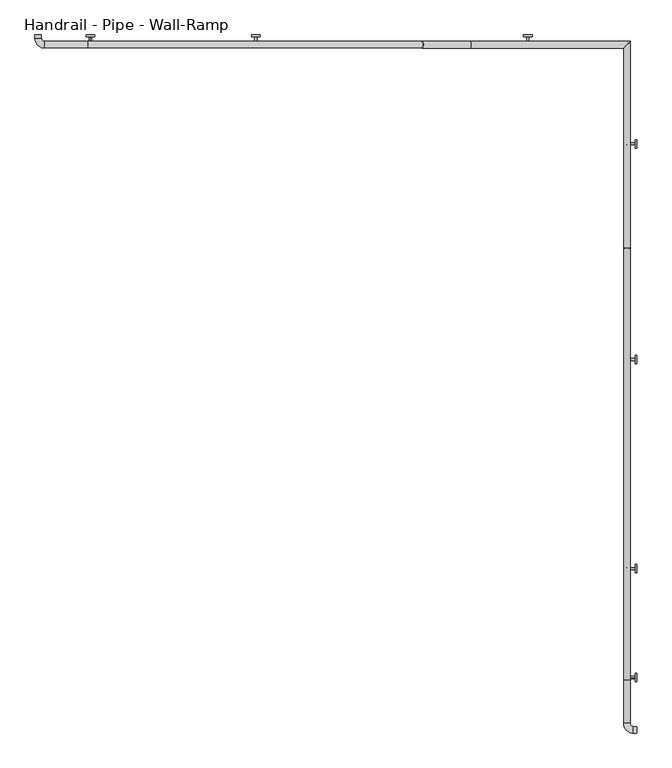
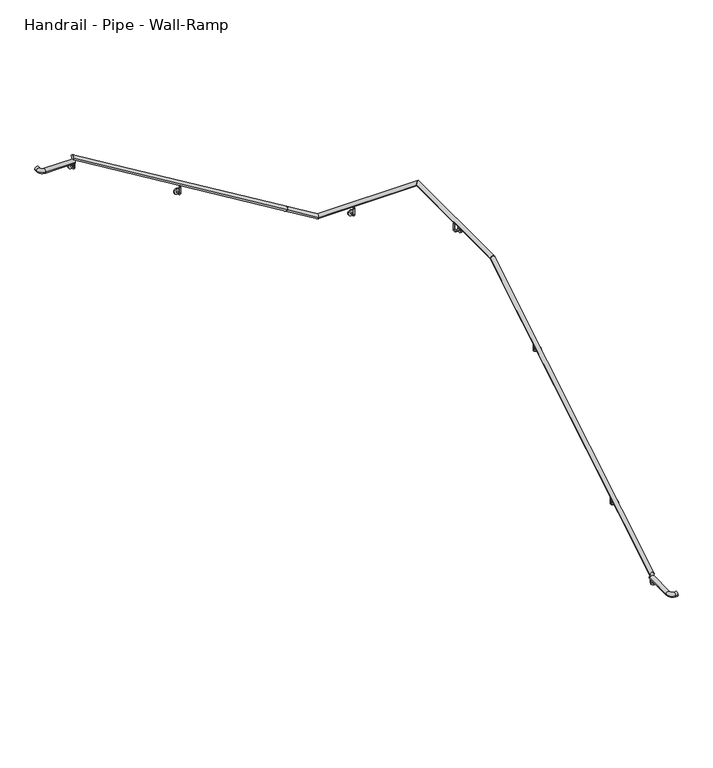
"""IFC4 building model written with IfcOpenShell, lengths in millimetres: railing geometry, Handrail - Pipe - Wall-Ramp."""

import ifcopenshell
import ifcopenshell.guid

model = None  # the IFC model being written
_history = None  # IfcOwnerHistory: only IFC2X3 demands one
_inside = {}  # id of a spatial element -> (the spatial element, [elements in it])
_under = {}  # id of a project, library or spatial element -> (it, [spatial elements below it])
_declared = {}  # id of a project -> (the project, [libraries it declares])
_typed = {}  # id of a type object -> (the type object, [elements of that type])
_made_of = {}  # id of a material, layer set ... -> (it, [elements and type objects made of it])


def new_model(schema):
    """Start an empty IFC model of exactly this schema.

    Asked for "IFC4X3", IfcOpenShell would pick the latest addendum, in which some entities
    have other attributes; the version numbers below select the first issue.
    IFC2X3 requires an IfcOwnerHistory on every rooted entity: one is made here for all.
    """
    global model, _history
    if schema == "IFC4X3":
        model = ifcopenshell.file(schema_version=(4, 3, 0, 0))
    else:
        model = ifcopenshell.file(schema=schema)
    _inside.clear()
    _under.clear()
    _declared.clear()
    _typed.clear()
    _made_of.clear()
    _history = None
    if model.schema == "IFC2X3":
        org = make("IfcOrganization", Name="unknown")
        user = make(
            "IfcPersonAndOrganization",
            ThePerson=make("IfcPerson", FamilyName="unknown"),
            TheOrganization=org,
        )
        app = make(
            "IfcApplication",
            ApplicationDeveloper=org,
            Version="unknown",
            ApplicationFullName="unknown",
            ApplicationIdentifier="unknown",
        )
        _history = make(
            "IfcOwnerHistory",
            OwningUser=user,
            OwningApplication=app,
            ChangeAction="ADDED",
            CreationDate=0,
        )
    return model


def make(cls, **values):
    """One entity of the class cls with the attributes given. An attribute that is None is left unset."""
    return model.create_entity(
        cls, **{name: value for name, value in values.items() if value is not None}
    )


def rooted(cls, **values):
    """An entity with a GlobalId (a new one), such as an element, a storey or a relation."""
    return make(cls, GlobalId=ifcopenshell.guid.new(), OwnerHistory=_history, **values)


def si_unit(unit_type, name, prefix=None):
    """IfcSIUnit, for example si_unit("LENGTHUNIT", "METRE", prefix="MILLI")."""
    return make("IfcSIUnit", UnitType=unit_type, Prefix=prefix, Name=name)


def assignment(units):
    """IfcUnitAssignment: the units of a project."""
    return None if units is None else make("IfcUnitAssignment", Units=units)


def point(xyz):
    """IfcCartesianPoint."""
    return None if xyz is None else make("IfcCartesianPoint", Coordinates=xyz)


def direction(xyz):
    """IfcDirection."""
    return None if xyz is None else make("IfcDirection", DirectionRatios=xyz)


def frame(location, z_axis=None, x_axis=None):
    """IfcAxis2Placement3D, a coordinate frame: its origin and axes. An axis left out is left unset."""
    return make(
        "IfcAxis2Placement3D",
        Location=point(location),
        Axis=direction(z_axis),
        RefDirection=direction(x_axis),
    )


def frame_2d(location, x_axis=None):
    """IfcAxis2Placement2D, a coordinate frame in the plane: its origin and x axis."""
    return make(
        "IfcAxis2Placement2D", Location=point(location), RefDirection=direction(x_axis)
    )


def origin():
    """The frame at (0, 0, 0) with its axes left unset."""
    return frame((0.0, 0.0, 0.0))


def place(relative_to, where):
    """IfcLocalPlacement: puts the frame where relative to a parent placement (None: the world)."""
    return make(
        "IfcLocalPlacement", PlacementRelTo=relative_to, RelativePlacement=where
    )


def context(
    kind, dimensions, precision=None, world=None, true_north=None, identifier=None
):
    """IfcGeometricRepresentationContext, for example the 3D "Model" context."""
    return make(
        "IfcGeometricRepresentationContext",
        ContextIdentifier=identifier,
        ContextType=kind,
        CoordinateSpaceDimension=dimensions,
        Precision=precision,
        WorldCoordinateSystem=world,
        TrueNorth=true_north,
    )


def project(units=None, contexts=None):
    """IfcProject with its units and contexts."""
    return rooted(
        "IfcProject",
        Name="project",
        RepresentationContexts=contexts,
        UnitsInContext=assignment(units),
    )


def spatial(cls, under=None, at=None, **own):
    """A site, building, storey or space (cls), placed at a placement, below another one or the project."""
    s = rooted(cls, ObjectPlacement=at, **own)
    if under is not None:
        _under.setdefault(under.id(), (under, []))[1].append(s)
    return s


def circle_curve(where, radius):
    """IfcCircle in the frame where."""
    return make("IfcCircle", Position=where, Radius=radius)


def ellipse_curve(where, semi_axis1, semi_axis2):
    """IfcEllipse in the frame where."""
    return make(
        "IfcEllipse", Position=where, SemiAxis1=semi_axis1, SemiAxis2=semi_axis2
    )


def trimmed(basis, trim1, trim2, sense, master):
    """IfcTrimmedCurve: the piece of a basis curve between two trims."""
    return make(
        "IfcTrimmedCurve",
        BasisCurve=basis,
        Trim1=trim1,
        Trim2=trim2,
        SenseAgreement=sense,
        MasterRepresentation=master,
    )


def segment(curve, same_sense, transition):
    """IfcCompositeCurveSegment."""
    return make(
        "IfcCompositeCurveSegment",
        Transition=transition,
        SameSense=same_sense,
        ParentCurve=curve,
    )


def composite_curve(segments, self_intersect=None):
    """IfcCompositeCurve: segments joined end to end."""
    return make("IfcCompositeCurve", Segments=segments, SelfIntersect=self_intersect)


def outline(outer, holes=None, kind="AREA"):
    """IfcArbitraryClosedProfileDef: a profile drawn as a closed curve; with holes, ...WithVoids."""
    if holes is None:
        return make("IfcArbitraryClosedProfileDef", ProfileType=kind, OuterCurve=outer)
    return make(
        "IfcArbitraryProfileDefWithVoids",
        ProfileType=kind,
        OuterCurve=outer,
        InnerCurves=holes,
    )


def extrude(swept, where, along, depth):
    """IfcExtrudedAreaSolid: the profile swept, set in the frame where, extruded along a direction by depth."""
    return make(
        "IfcExtrudedAreaSolid",
        SweptArea=swept,
        Position=where,
        ExtrudedDirection=direction(along),
        Depth=depth,
    )


def shape(context_of_items, identifier, shape_type, items):
    """IfcShapeRepresentation: the items that make up one representation, for example the "Body"."""
    return make(
        "IfcShapeRepresentation",
        ContextOfItems=context_of_items,
        RepresentationIdentifier=identifier,
        RepresentationType=shape_type,
        Items=items,
    )


def source(mapping_origin, context_of_items, identifier, shape_type, items):
    """IfcRepresentationMap: a shape defined once, which mapped items show again and again."""
    return make(
        "IfcRepresentationMap",
        MappingOrigin=mapping_origin,
        MappedRepresentation=shape(context_of_items, identifier, shape_type, items),
    )


def transform(
    local_origin,
    x_axis=None,
    y_axis=None,
    z_axis=None,
    scale=None,
    scale2=None,
    scale3=None,
    uniform=True,
):
    """IfcCartesianTransformationOperator3D, or its non-uniform kind. x_axis, y_axis, z_axis: its Axis1, 2, 3."""
    if uniform:
        return make(
            "IfcCartesianTransformationOperator3D",
            Axis1=direction(x_axis),
            Axis2=direction(y_axis),
            LocalOrigin=point(local_origin),
            Scale=scale,
            Axis3=direction(z_axis),
        )
    return make(
        "IfcCartesianTransformationOperator3DnonUniform",
        Axis1=direction(x_axis),
        Axis2=direction(y_axis),
        LocalOrigin=point(local_origin),
        Scale=scale,
        Axis3=direction(z_axis),
        Scale2=scale2,
        Scale3=scale3,
    )


def mapped(mapping_source, mapping_target):
    """IfcMappedItem: shows the shape of a source again, moved by a transform."""
    return make(
        "IfcMappedItem", MappingSource=mapping_source, MappingTarget=mapping_target
    )


def made_of(thing, what):
    """Note that an element or type object is made of a material, layer set ...; save() writes the relation."""
    if what is not None:
        _made_of.setdefault(what.id(), (what, []))[1].append(thing)
    return thing


def element(
    cls,
    number,
    at=None,
    inside=None,
    cuts=None,
    type_object=None,
    material=None,
    context=None,
    identifier="Body",
    shape_type=None,
    held_by="IfcProductDefinitionShape",
    body=None,
    shapes=None,
    **own,
):
    """One element of the class cls, such as IfcWall. Its Tag is "e" and its number.

    at: its placement. inside: the storey or other place that contains it. cuts: it is an
    opening in that element (IfcRelVoidsElement). A single representation is given by context,
    identifier, shape_type and body (its items); several are given by shapes. held_by: the class
    of the entity that holds the representations. save() writes the other relations.
    """
    e = rooted(cls, Tag="e%d" % number, ObjectPlacement=at, **own)
    if body is not None:
        shapes = [shape(context, identifier, shape_type, body)]
    if shapes is not None:
        e.Representation = make(held_by, Representations=shapes)
    if inside is not None:
        _inside.setdefault(inside.id(), (inside, []))[1].append(e)
    if cuts is not None:
        rooted(
            "IfcRelVoidsElement", RelatingBuildingElement=cuts, RelatedOpeningElement=e
        )
    if type_object is not None:
        _typed.setdefault(type_object.id(), (type_object, []))[1].append(e)
    return made_of(e, material)


def aggregate(whole, parts):
    """IfcRelAggregates: a whole, such as a stair, and the parts it consists of."""
    return rooted("IfcRelAggregates", RelatingObject=whole, RelatedObjects=parts)


def save(model, path):
    """Write the relations noted so far, then the file.

    IfcRelAggregates (storeys below a building ...), IfcRelContainedInSpatialStructure (elements
    in a storey), IfcRelDefinesByType, IfcRelAssociatesMaterial and IfcRelDeclares: one each for
    every whole, place, type object, material and project.
    """
    for whole, parts in _under.values():
        aggregate(whole, parts)
    for where, things in _inside.values():
        rooted(
            "IfcRelContainedInSpatialStructure",
            RelatedElements=things,
            RelatingStructure=where,
        )
    for kind, things in _typed.values():
        rooted("IfcRelDefinesByType", RelatedObjects=things, RelatingType=kind)
    for what, things in _made_of.values():
        rooted("IfcRelAssociatesMaterial", RelatedObjects=things, RelatingMaterial=what)
    for by, libraries in _declared.values():
        rooted("IfcRelDeclares", RelatingContext=by, RelatedDefinitions=libraries)
    model.write(path)


def plane_surface(at):
    """IfcPlane: the flat surface through the origin of the frame at, square to its z axis."""
    return make("IfcPlane", Position=at)


def cylinder_surface(at, radius):
    """IfcCylindricalSurface: all points at the distance radius from the z axis of the frame at."""
    return make("IfcCylindricalSurface", Position=at, Radius=radius)


def revolved_surface(curve, axis_point, axis_direction):
    """IfcSurfaceOfRevolution: the curve turned about the line through axis_point along axis_direction."""
    return make(
        "IfcSurfaceOfRevolution",
        SweptCurve=make("IfcArbitraryOpenProfileDef", ProfileType="CURVE", Curve=curve),
        AxisPosition=make("IfcAxis1Placement", Location=point(axis_point), Axis=direction(axis_direction)),
    )


def advanced_brep(points, edges, surfaces, faces):
    """IfcAdvancedBrep: a solid bounded by faces that lie on surfaces and meet in shared edges.

    An edge is (start, end): straight between two places in points (the first is 0);
    or (start, end, curve); or (start, end, curve, False) where it runs against its curve.
    A face is (place in surfaces, loops), or (place, loops, False) where it looks against
    its surface's normal. A loop lists edges by number (the first is 1), with a minus sign
    where the edge is run from its end to its start. The first loop is the outer one.
    """
    corners = [point(p) for p in points]
    vertices = [make("IfcVertexPoint", VertexGeometry=c) for c in corners]
    made = []
    for start, end, *more in edges:
        made.append(
            make(
                "IfcEdgeCurve",
                EdgeStart=vertices[start],
                EdgeEnd=vertices[end],
                EdgeGeometry=more[0] if more else make("IfcPolyline", Points=[corners[start], corners[end]]),
                SameSense=more[1] if len(more) > 1 else True,
            )
        )
    hull = []
    for where, loops, *sense in faces:
        bounds = []
        for j, loop in enumerate(loops):
            ring = [make("IfcOrientedEdge", EdgeElement=made[abs(k) - 1], Orientation=k > 0) for k in loop]
            bounds.append(
                make(
                    "IfcFaceOuterBound" if j == 0 else "IfcFaceBound",
                    Bound=make("IfcEdgeLoop", EdgeList=ring),
                    Orientation=True,
                )
            )
        hull.append(make("IfcAdvancedFace", Bounds=bounds, FaceSurface=surfaces[where], SameSense=sense[0] if sense else True))
    return make("IfcAdvancedBrep", Outer=make("IfcClosedShell", CfsFaces=hull))


def handrail_pipe_wall_ramp_3ec7286e(model_context):
    return source(origin(), model_context, "Body", "SolidModel", [
        advanced_brep(
        [(-6920.3581077, -11181.433999, 1061.4577857), (-6882.2581077, -11181.433999, 1061.4577857), (-6920.3581077, -8661.5118455, 2588.6833333), (-6882.2581077, -8661.5118455, 2588.6833333)],
        [
            (0, 1, ellipse_curve(frame((-6901.3081077, -11181.433999, 1061.4577857), z_axis=(0.0, -1.0, 0.0), x_axis=(0.0, 0.0, -1.0)), 22.2755476, 19.05)),
            (1, 0, ellipse_curve(frame((-6901.3081077, -11181.433999, 1061.4577857), z_axis=(0.0, -1.0, 0.0), x_axis=(0.0, 0.0, -1.0)), 22.2755476, 19.05)),
            (2, 3, ellipse_curve(frame((-6901.3081077, -8661.5118455, 2588.6833333), z_axis=(0.0, 0.963119367356418, 0.26907449567540415), x_axis=(0.0, 0.26907449567540404, -0.9631193673564179)), 19.7794797, 19.05)),
            (3, 2, ellipse_curve(frame((-6901.3081077, -8661.5118455, 2588.6833333), z_axis=(0.0, 0.963119367356418, 0.26907449567540415), x_axis=(0.0, 0.26907449567540404, -0.9631193673564179)), 19.7794797, 19.05)),
            (0, 2),
            (3, 1),
        ],
        [
            plane_surface(frame((-6901.3081077, -11181.433999, 1083.7333333), z_axis=(0.0, -1.0, 0.0), x_axis=(0.0, 0.0, 1.0))),
            plane_surface(frame((-6901.3081077, -8666.833999, 2607.7333333), z_axis=(0.0, 0.963119367356418, 0.26907449567540415), x_axis=(1.0, 0.0, 0.0))),
            cylinder_surface(frame((-6901.3081077, -11171.5603513, 1067.4418146), z_axis=(0.0, -0.8551978315540538, -0.518301716093285), x_axis=(1.0, 0.0, 0.0)), 19.05),
        ],
        [
            (0, [[1, 2]]),
            (1, [[3, 4]]),
            (2, [[-1, 5, -4, 6]]),
            (2, [[-2, -6, -3, -5]]),
        ],
    ),
        advanced_brep(
        [(-6920.3581077, -8661.5118455, 2588.6833333), (-6882.2581077, -8661.5118455, 2588.6833333), (-6920.3581077, -7498.433999, 2588.6833333), (-6882.2581077, -7460.333999, 2588.6833333)],
        [
            (0, 1, ellipse_curve(frame((-6901.3081077, -8661.5118455, 2588.6833333), z_axis=(0.0, -0.963119367356418, -0.26907449567540415), x_axis=(0.0, -0.2690744956754042, 0.963119367356418)), 19.7794797, 19.05)),
            (1, 0, ellipse_curve(frame((-6901.3081077, -8661.5118455, 2588.6833333), z_axis=(0.0, -0.963119367356418, -0.26907449567540415), x_axis=(0.0, -0.2690744956754042, 0.963119367356418)), 19.7794797, 19.05)),
            (2, 3, ellipse_curve(frame((-6901.3081077, -7479.383999, 2588.6833333), z_axis=(-0.7071067811865462, 0.7071067811865488, 0.0), x_axis=(-0.7071067811865488, -0.7071067811865462, 0.0)), 26.9407684, 19.05)),
            (3, 2, ellipse_curve(frame((-6901.3081077, -7479.383999, 2588.6833333), z_axis=(-0.7071067811865462, 0.7071067811865488, 0.0), x_axis=(-0.7071067811865488, -0.7071067811865462, 0.0)), 26.9407684, 19.05)),
            (0, 2),
            (3, 1),
        ],
        [
            plane_surface(frame((-6901.3081077, -8666.833999, 2607.7333333), z_axis=(0.0, -0.963119367356418, -0.26907449567540415), x_axis=(1.0, 0.0, 0.0))),
            plane_surface(frame((-6901.3081077, -7479.383999, 2607.7333333), z_axis=(-0.7071067811865462, 0.7071067811865488, 0.0), x_axis=(0.7071067811865488, 0.7071067811865462, 0.0))),
            cylinder_surface(frame((-6901.3081077, -8666.833999, 2588.6833333), z_axis=(0.0, -1.0, 0.0), x_axis=(1.0, 0.0, 0.0)), 19.05),
        ],
        [
            (0, [[1, 2]]),
            (1, [[3, 4]]),
            (2, [[-1, 5, -4, 6]]),
            (2, [[-2, -6, -3, -5]]),
        ],
    ),
        advanced_brep(
        [(-6920.3581077, -7498.433999, 2588.6833333), (-6882.2581077, -7460.333999, 2588.6833333), (-7814.6802613, -7498.433999, 2588.6833333), (-7814.6802613, -7460.333999, 2588.6833333), (-8098.6317554, -7498.433999, 2760.775148), (-8098.6317554, -7460.333999, 2760.775148)],
        [
            (0, 1, ellipse_curve(frame((-6901.3081077, -7479.383999, 2588.6833333), z_axis=(0.7071067811865462, -0.7071067811865488, 0.0), x_axis=(0.7071067811865488, 0.7071067811865462, 0.0)), 26.9407684, 19.05)),
            (1, 0, ellipse_curve(frame((-6901.3081077, -7479.383999, 2588.6833333), z_axis=(0.7071067811865462, -0.7071067811865488, 0.0), x_axis=(0.7071067811865488, 0.7071067811865462, 0.0)), 26.9407684, 19.05)),
            (0, 2),
            (2, 3, ellipse_curve(frame((-7814.6802613, -7479.383999, 2588.6833333), z_axis=(0.9631193673564179, 0.0, -0.2690744956754043), x_axis=(0.2690744956754048, 0.0, 0.9631193673564179)), 19.7794797, 19.05)),
            (3, 1),
            (3, 2, ellipse_curve(frame((-7814.6802613, -7479.383999, 2588.6833333), z_axis=(0.9631193673564179, 0.0, -0.2690744956754043), x_axis=(0.2690744956754048, 0.0, 0.9631193673564179)), 19.7794797, 19.05)),
            (4, 5, circle_curve(frame((-8098.6317554, -7479.383999, 2760.775148), z_axis=(-0.8551978315540536, 0.0, 0.5183017160932853), x_axis=(0.0, 1.0, 0.0)), 19.05)),
            (5, 4, circle_curve(frame((-8098.6317554, -7479.383999, 2760.775148), z_axis=(-0.8551978315540536, 0.0, 0.5183017160932853), x_axis=(0.0, 1.0, 0.0)), 19.05)),
            (2, 4),
            (5, 3),
        ],
        [
            plane_surface(frame((-6901.3081077, -7479.383999, 2607.7333333), z_axis=(0.7071067811865462, -0.7071067811865488, 0.0), x_axis=(0.7071067811865488, 0.7071067811865462, 0.0))),
            cylinder_surface(frame((-6901.3081077, -7479.383999, 2588.6833333), z_axis=(1.0, 0.0, 0.0), x_axis=(0.0, 1.0, 0.0)), 19.05),
            plane_surface(frame((-8088.7581077, -7479.383999, 2777.0666667), z_axis=(-0.8551978315540536, 0.0, 0.5183017160932853), x_axis=(0.5183017160932853, 0.0, 0.8551978315540536))),
            cylinder_surface(frame((-7819.2317554, -7479.383999, 2591.4418146), z_axis=(0.8551978315540536, 0.0, -0.5183017160932853), x_axis=(0.0, 1.0, 0.0)), 19.05),
        ],
        [
            (0, [[1, 2]]),
            (1, [[-1, 3, 4, 5]]),
            (1, [[-2, -5, 6, -3]]),
            (2, [[7, 8]]),
            (3, [[-4, 9, -8, 10]]),
            (3, [[-6, -10, -7, -9]]),
        ],
    ),
        advanced_brep(
        [(-8098.6317554, -7498.433999, 2760.775148), (-8098.6317554, -7460.333999, 2760.775148), (-10044.5581077, -7498.433999, 3940.1244524), (-10044.5581077, -7460.333999, 3940.1244524)],
        [
            (0, 1, circle_curve(frame((-8098.6317554, -7479.383999, 2760.775148), z_axis=(0.8551978315540537, 0.0, -0.5183017160932851), x_axis=(0.0, 1.0, 0.0)), 19.05)),
            (1, 0, circle_curve(frame((-8098.6317554, -7479.383999, 2760.775148), z_axis=(0.8551978315540537, 0.0, -0.5183017160932851), x_axis=(0.0, 1.0, 0.0)), 19.05)),
            (2, 3, ellipse_curve(frame((-10044.5581077, -7479.383999, 3940.1244524), z_axis=(-1.0, 0.0, 0.0), x_axis=(0.0, 0.0, -1.0)), 22.2755476, 19.05)),
            (3, 2, ellipse_curve(frame((-10044.5581077, -7479.383999, 3940.1244524), z_axis=(-1.0, 0.0, 0.0), x_axis=(0.0, 0.0, -1.0)), 22.2755476, 19.05)),
            (0, 2),
            (3, 1),
        ],
        [
            plane_surface(frame((-8088.7581077, -7479.383999, 2777.0666667), z_axis=(0.8551978315540538, 0.0, -0.5183017160932851), x_axis=(0.5183017160932851, 0.0, 0.8551978315540538))),
            plane_surface(frame((-10044.5581077, -7479.383999, 3962.4), z_axis=(-1.0, 0.0, 0.0), x_axis=(0.0, -1.0, 0.0))),
            cylinder_surface(frame((-8098.6317554, -7479.383999, 2760.775148), z_axis=(0.8551978315540537, 0.0, -0.5183017160932851), x_axis=(0.0, 1.0, 0.0)), 19.05),
        ],
        [
            (0, [[1, 2]]),
            (1, [[3, 4]]),
            (2, [[-1, 5, -4, 6]]),
            (2, [[-2, -6, -3, -5]]),
        ],
    ),
        advanced_brep(
        [(-9060.3081077, -7479.383999, 3312.5833333), (-9073.0081077, -7479.383999, 3312.5833333), (-9060.3081077, -7479.383999, 3255.4333333), (-9073.0081077, -7479.383999, 3255.4333333), (-9073.0081077, -7460.333999, 3236.3833333), (-9060.3081077, -7460.333999, 3236.3833333), (-9060.3081077, -7431.758999, 3236.3833333), (-9073.0081077, -7431.758999, 3236.3833333)],
        [
            (0, 1, circle_curve(frame((-9066.6581077, -7479.383999, 3312.5833333), z_axis=(0.0, 0.0, 1.0), x_axis=(-1.0, 0.0, 0.0)), 6.35)),
            (1, 0, circle_curve(frame((-9066.6581077, -7479.383999, 3312.5833333), z_axis=(0.0, 0.0, 1.0), x_axis=(-1.0, 0.0, 0.0)), 6.35)),
            (0, 2),
            (2, 3, circle_curve(frame((-9066.6581077, -7479.383999, 3255.4333333), z_axis=(0.0, 0.0, 1.0), x_axis=(-1.0, 0.0, 0.0)), 6.35)),
            (3, 1),
            (3, 2, circle_curve(frame((-9066.6581077, -7479.383999, 3255.4333333), z_axis=(0.0, 0.0, 1.0), x_axis=(-1.0, 0.0, 0.0)), 6.35)),
            (4, 3, circle_curve(frame((-9073.0081077, -7460.333999, 3255.4333333), z_axis=(-1.0, 0.0, 0.0), x_axis=(0.0, -1.0, 0.0)), 19.05)),
            (2, 5, circle_curve(frame((-9060.3081077, -7460.333999, 3255.4333333), z_axis=(1.0, 0.0, 0.0), x_axis=(0.0, -1.0, 0.0)), 19.05)),
            (5, 4, circle_curve(frame((-9066.6581077, -7460.333999, 3236.3833333), z_axis=(0.0, -1.0, 0.0), x_axis=(-1.0, 0.0, 0.0)), 6.35)),
            (4, 5, circle_curve(frame((-9066.6581077, -7460.333999, 3236.3833333), z_axis=(0.0, -1.0, 0.0), x_axis=(-1.0, 0.0, 0.0)), 6.35)),
            (6, 7, circle_curve(frame((-9066.6581077, -7431.758999, 3236.3833333), z_axis=(0.0, 1.0, 0.0), x_axis=(-1.0, 0.0, 0.0)), 6.35)),
            (7, 6, circle_curve(frame((-9066.6581077, -7431.758999, 3236.3833333), z_axis=(0.0, 1.0, 0.0), x_axis=(-1.0, 0.0, 0.0)), 6.35)),
            (5, 6),
            (7, 4),
        ],
        [
            plane_surface(frame((-9073.0081077, -7479.383999, 3312.5833333), z_axis=(0.0, 0.0, 1.0), x_axis=(0.0, 1.0, 0.0))),
            cylinder_surface(frame((-9066.6581077, -7479.383999, 3312.5833333), z_axis=(0.0, 0.0, 1.0), x_axis=(-1.0, 0.0, 0.0)), 6.35),
            revolved_surface(trimmed(ellipse_curve(frame((-9066.6581077, -7479.383999, 3255.4333333), z_axis=(0.0, 0.0, 1.0), x_axis=(-1.0, 0.0, 0.0)), 6.35, 6.35), [point((-9060.3081077, -7479.383999, 3255.4333333))], [point((-9073.0081077, -7479.383999, 3255.4333333))], True, "CARTESIAN"), (-9066.6581077, -7460.333999, 3255.4333333), (1.0, 0.0, 0.0)),
            revolved_surface(trimmed(ellipse_curve(frame((-9066.6581077, -7479.383999, 3255.4333333), z_axis=(0.0, 0.0, 1.0), x_axis=(-1.0, 0.0, 0.0)), 6.35, 6.35), [point((-9073.0081077, -7479.383999, 3255.4333333))], [point((-9060.3081077, -7479.383999, 3255.4333333))], True, "CARTESIAN"), (-9066.6581077, -7460.333999, 3255.4333333), (1.0, 0.0, 0.0)),
            plane_surface(frame((-9066.6581077, -7431.758999, 3230.0333333), z_axis=(0.0, 1.0, 0.0), x_axis=(-1.0, 0.0, 0.0))),
            cylinder_surface(frame((-9066.6581077, -7460.333999, 3236.3833333), z_axis=(0.0, -1.0, 0.0), x_axis=(-1.0, 0.0, 0.0)), 6.35),
        ],
        [
            (0, [[1, 2]]),
            (1, [[-1, 3, 4, 5]]),
            (1, [[-2, -5, 6, -3]]),
            (2, [[7, -4, 8, 9]]),
            (3, [[-8, -6, -7, 10]]),
            (4, [[11, 12]]),
            (5, [[-9, 13, -12, 14]]),
            (5, [[-10, -14, -11, -13]]),
        ],
    ),
        extrude(outline(composite_curve([segment(trimmed(circle_curve(frame_2d((3236.3833333, -9066.6581077)), 25.4), [point((3236.3833333, -9092.0581077))], [point((3236.3833333, -9041.2581077))], False, "CARTESIAN"), True, "CONTINUOUS"), segment(trimmed(circle_curve(frame_2d((3236.3833333, -9066.6581077)), 25.4), [point((3236.3833333, -9041.2581077))], [point((3236.3833333, -9092.0581077))], False, "CARTESIAN"), True, "CONTINUOUS")], self_intersect=False)), frame((0.0, -7431.758999, 0.0), z_axis=(0.0, 1.0, 0.0), x_axis=(0.0, 0.0, 1.0)), (0.0, 0.0, 1.0), 9.525),
        advanced_brep(
        [(-7472.8081077, -7479.383999, 2550.5833333), (-7485.5081077, -7479.383999, 2550.5833333), (-7472.8081077, -7479.383999, 2493.4333333), (-7485.5081077, -7479.383999, 2493.4333333), (-7485.5081077, -7460.333999, 2474.3833333), (-7472.8081077, -7460.333999, 2474.3833333), (-7472.8081077, -7431.758999, 2474.3833333), (-7485.5081077, -7431.758999, 2474.3833333)],
        [
            (0, 1, circle_curve(frame((-7479.1581077, -7479.383999, 2550.5833333), z_axis=(0.0, 0.0, 1.0), x_axis=(-1.0, 0.0, 0.0)), 6.35)),
            (1, 0, circle_curve(frame((-7479.1581077, -7479.383999, 2550.5833333), z_axis=(0.0, 0.0, 1.0), x_axis=(-1.0, 0.0, 0.0)), 6.35)),
            (0, 2),
            (2, 3, circle_curve(frame((-7479.1581077, -7479.383999, 2493.4333333), z_axis=(0.0, 0.0, 1.0), x_axis=(-1.0, 0.0, 0.0)), 6.35)),
            (3, 1),
            (3, 2, circle_curve(frame((-7479.1581077, -7479.383999, 2493.4333333), z_axis=(0.0, 0.0, 1.0), x_axis=(-1.0, 0.0, 0.0)), 6.35)),
            (4, 3, circle_curve(frame((-7485.5081077, -7460.333999, 2493.4333333), z_axis=(-1.0, 0.0, 0.0), x_axis=(0.0, -1.0, 0.0)), 19.05)),
            (2, 5, circle_curve(frame((-7472.8081077, -7460.333999, 2493.4333333), z_axis=(1.0, 0.0, 0.0), x_axis=(0.0, -1.0, 0.0)), 19.05)),
            (5, 4, circle_curve(frame((-7479.1581077, -7460.333999, 2474.3833333), z_axis=(0.0, -1.0, 0.0), x_axis=(-1.0, 0.0, 0.0)), 6.35)),
            (4, 5, circle_curve(frame((-7479.1581077, -7460.333999, 2474.3833333), z_axis=(0.0, -1.0, 0.0), x_axis=(-1.0, 0.0, 0.0)), 6.35)),
            (6, 7, circle_curve(frame((-7479.1581077, -7431.758999, 2474.3833333), z_axis=(0.0, 1.0, 0.0), x_axis=(-1.0, 0.0, 0.0)), 6.35)),
            (7, 6, circle_curve(frame((-7479.1581077, -7431.758999, 2474.3833333), z_axis=(0.0, 1.0, 0.0), x_axis=(-1.0, 0.0, 0.0)), 6.35)),
            (5, 6),
            (7, 4),
        ],
        [
            plane_surface(frame((-7485.5081077, -7479.383999, 2550.5833333), z_axis=(0.0, 0.0, 1.0), x_axis=(0.0, 1.0, 0.0))),
            cylinder_surface(frame((-7479.1581077, -7479.383999, 2550.5833333), z_axis=(0.0, 0.0, 1.0), x_axis=(-1.0, 0.0, 0.0)), 6.35),
            revolved_surface(trimmed(ellipse_curve(frame((-7479.1581077, -7479.383999, 2493.4333333), z_axis=(0.0, 0.0, 1.0), x_axis=(-1.0, 0.0, 0.0)), 6.35, 6.35), [point((-7472.8081077, -7479.383999, 2493.4333333))], [point((-7485.5081077, -7479.383999, 2493.4333333))], True, "CARTESIAN"), (-7479.1581077, -7460.333999, 2493.4333333), (1.0, 0.0, 0.0)),
            revolved_surface(trimmed(ellipse_curve(frame((-7479.1581077, -7479.383999, 2493.4333333), z_axis=(0.0, 0.0, 1.0), x_axis=(-1.0, 0.0, 0.0)), 6.35, 6.35), [point((-7485.5081077, -7479.383999, 2493.4333333))], [point((-7472.8081077, -7479.383999, 2493.4333333))], True, "CARTESIAN"), (-7479.1581077, -7460.333999, 2493.4333333), (1.0, 0.0, 0.0)),
            plane_surface(frame((-7479.1581077, -7431.758999, 2468.0333333), z_axis=(0.0, 1.0, 0.0), x_axis=(-1.0, 0.0, 0.0))),
            cylinder_surface(frame((-7479.1581077, -7460.333999, 2474.3833333), z_axis=(0.0, -1.0, 0.0), x_axis=(-1.0, 0.0, 0.0)), 6.35),
        ],
        [
            (0, [[1, 2]]),
            (1, [[-1, 3, 4, 5]]),
            (1, [[-2, -5, 6, -3]]),
            (2, [[7, -4, 8, 9]]),
            (3, [[-8, -6, -7, 10]]),
            (4, [[11, 12]]),
            (5, [[-9, 13, -12, 14]]),
            (5, [[-10, -14, -11, -13]]),
        ],
    ),
        extrude(outline(composite_curve([segment(trimmed(circle_curve(frame_2d((2474.3833333, -7479.1581077)), 25.4), [point((2474.3833333, -7504.5581077))], [point((2474.3833333, -7453.7581077))], False, "CARTESIAN"), True, "CONTINUOUS"), segment(trimmed(circle_curve(frame_2d((2474.3833333, -7479.1581077)), 25.4), [point((2474.3833333, -7453.7581077))], [point((2474.3833333, -7504.5581077))], False, "CARTESIAN"), True, "CONTINUOUS")], self_intersect=False)), frame((0.0, -7431.758999, 0.0), z_axis=(0.0, 1.0, 0.0), x_axis=(0.0, 0.0, 1.0)), (0.0, 0.0, 1.0), 9.525),
        advanced_brep(
        [(-6901.3081077, -8063.583999, 2550.5833333), (-6901.3081077, -8050.883999, 2550.5833333), (-6901.3081077, -8063.583999, 2493.4333333), (-6901.3081077, -8050.883999, 2493.4333333), (-6882.2581077, -8050.883999, 2474.3833333), (-6882.2581077, -8063.583999, 2474.3833333), (-6853.6831077, -8063.583999, 2474.3833333), (-6853.6831077, -8050.883999, 2474.3833333)],
        [
            (0, 1, circle_curve(frame((-6901.3081077, -8057.233999, 2550.5833333), z_axis=(0.0, 0.0, 1.0), x_axis=(0.0, 1.0, 0.0)), 6.35)),
            (1, 0, circle_curve(frame((-6901.3081077, -8057.233999, 2550.5833333), z_axis=(0.0, 0.0, 1.0), x_axis=(0.0, 1.0, 0.0)), 6.35)),
            (0, 2),
            (2, 3, circle_curve(frame((-6901.3081077, -8057.233999, 2493.4333333), z_axis=(0.0, 0.0, 1.0), x_axis=(0.0, 1.0, 0.0)), 6.35)),
            (3, 1),
            (3, 2, circle_curve(frame((-6901.3081077, -8057.233999, 2493.4333333), z_axis=(0.0, 0.0, 1.0), x_axis=(0.0, 1.0, 0.0)), 6.35)),
            (4, 3, circle_curve(frame((-6882.2581077, -8050.883999, 2493.4333333), z_axis=(0.0, 1.0, 0.0), x_axis=(-1.0, 0.0, 0.0)), 19.05)),
            (2, 5, circle_curve(frame((-6882.2581077, -8063.583999, 2493.4333333), z_axis=(0.0, -1.0, 0.0), x_axis=(-1.0, 0.0, 0.0)), 19.05)),
            (5, 4, circle_curve(frame((-6882.2581077, -8057.233999, 2474.3833333), z_axis=(-1.0, 0.0, 0.0), x_axis=(0.0, 1.0, 0.0)), 6.35)),
            (4, 5, circle_curve(frame((-6882.2581077, -8057.233999, 2474.3833333), z_axis=(-1.0, 0.0, 0.0), x_axis=(0.0, 1.0, 0.0)), 6.35)),
            (6, 7, circle_curve(frame((-6853.6831077, -8057.233999, 2474.3833333), z_axis=(1.0, 0.0, 0.0), x_axis=(0.0, 1.0, 0.0)), 6.35)),
            (7, 6, circle_curve(frame((-6853.6831077, -8057.233999, 2474.3833333), z_axis=(1.0, 0.0, 0.0), x_axis=(0.0, 1.0, 0.0)), 6.35)),
            (5, 6),
            (7, 4),
        ],
        [
            plane_surface(frame((-6901.3081077, -8050.883999, 2550.5833333), z_axis=(0.0, 0.0, 1.0), x_axis=(1.0, 0.0, 0.0))),
            cylinder_surface(frame((-6901.3081077, -8057.233999, 2550.5833333), z_axis=(0.0, 0.0, 1.0), x_axis=(0.0, 1.0, 0.0)), 6.35),
            revolved_surface(trimmed(ellipse_curve(frame((-6901.3081077, -8057.233999, 2493.4333333), z_axis=(0.0, 0.0, 1.0), x_axis=(0.0, 1.0, 0.0)), 6.35, 6.35), [point((-6901.3081077, -8063.583999, 2493.4333333))], [point((-6901.3081077, -8050.883999, 2493.4333333))], True, "CARTESIAN"), (-6882.2581077, -8057.233999, 2493.4333333), (0.0, -1.0, 0.0)),
            revolved_surface(trimmed(ellipse_curve(frame((-6901.3081077, -8057.233999, 2493.4333333), z_axis=(0.0, 0.0, 1.0), x_axis=(0.0, 1.0, 0.0)), 6.35, 6.35), [point((-6901.3081077, -8050.883999, 2493.4333333))], [point((-6901.3081077, -8063.583999, 2493.4333333))], True, "CARTESIAN"), (-6882.2581077, -8057.233999, 2493.4333333), (0.0, -1.0, 0.0)),
            plane_surface(frame((-6853.6831077, -8057.233999, 2468.0333333), z_axis=(1.0, 0.0, 0.0), x_axis=(0.0, 1.0, 0.0))),
            cylinder_surface(frame((-6882.2581077, -8057.233999, 2474.3833333), z_axis=(-1.0, 0.0, 0.0), x_axis=(0.0, 1.0, 0.0)), 6.35),
        ],
        [
            (0, [[1, 2]]),
            (1, [[-1, 3, 4, 5]]),
            (1, [[-2, -5, 6, -3]]),
            (2, [[7, -4, 8, 9]]),
            (3, [[-8, -6, -7, 10]]),
            (4, [[11, 12]]),
            (5, [[-9, 13, -12, 14]]),
            (5, [[-10, -14, -11, -13]]),
        ],
    ),
        extrude(outline(composite_curve([segment(trimmed(circle_curve(frame_2d((-8057.233999, 2474.3833333)), 25.4), [point((-8031.833999, 2474.3833333))], [point((-8082.633999, 2474.3833333))], False, "CARTESIAN"), True, "CONTINUOUS"), segment(trimmed(circle_curve(frame_2d((-8057.233999, 2474.3833333)), 25.4), [point((-8082.633999, 2474.3833333))], [point((-8031.833999, 2474.3833333))], False, "CARTESIAN"), True, "CONTINUOUS")], self_intersect=False)), frame((-6853.6831077, 0.0, 0.0), z_axis=(1.0, 0.0, 0.0), x_axis=(0.0, 1.0, 0.0)), (0.0, 0.0, 1.0), 9.525),
        advanced_brep(
        [(-6901.3081077, -9320.883999, 2158.0378788), (-6901.3081077, -9308.183999, 2158.0378788), (-6901.3081077, -9320.883999, 2100.8878788), (-6901.3081077, -9308.183999, 2100.8878788), (-6882.2581077, -9308.183999, 2081.8378788), (-6882.2581077, -9320.883999, 2081.8378788), (-6853.6831077, -9320.883999, 2081.8378788), (-6853.6831077, -9308.183999, 2081.8378788)],
        [
            (0, 1, circle_curve(frame((-6901.3081077, -9314.533999, 2158.0378788), z_axis=(0.0, 0.0, 1.0), x_axis=(0.0, 1.0, 0.0)), 6.35)),
            (1, 0, circle_curve(frame((-6901.3081077, -9314.533999, 2158.0378788), z_axis=(0.0, 0.0, 1.0), x_axis=(0.0, 1.0, 0.0)), 6.35)),
            (0, 2),
            (2, 3, circle_curve(frame((-6901.3081077, -9314.533999, 2100.8878788), z_axis=(0.0, 0.0, 1.0), x_axis=(0.0, 1.0, 0.0)), 6.35)),
            (3, 1),
            (3, 2, circle_curve(frame((-6901.3081077, -9314.533999, 2100.8878788), z_axis=(0.0, 0.0, 1.0), x_axis=(0.0, 1.0, 0.0)), 6.35)),
            (4, 3, circle_curve(frame((-6882.2581077, -9308.183999, 2100.8878788), z_axis=(0.0, 1.0, 0.0), x_axis=(-1.0, 0.0, 0.0)), 19.05)),
            (2, 5, circle_curve(frame((-6882.2581077, -9320.883999, 2100.8878788), z_axis=(0.0, -1.0, 0.0), x_axis=(-1.0, 0.0, 0.0)), 19.05)),
            (5, 4, circle_curve(frame((-6882.2581077, -9314.533999, 2081.8378788), z_axis=(-1.0, 0.0, 0.0), x_axis=(0.0, 1.0, 0.0)), 6.35)),
            (4, 5, circle_curve(frame((-6882.2581077, -9314.533999, 2081.8378788), z_axis=(-1.0, 0.0, 0.0), x_axis=(0.0, 1.0, 0.0)), 6.35)),
            (6, 7, circle_curve(frame((-6853.6831077, -9314.533999, 2081.8378788), z_axis=(1.0, 0.0, 0.0), x_axis=(0.0, 1.0, 0.0)), 6.35)),
            (7, 6, circle_curve(frame((-6853.6831077, -9314.533999, 2081.8378788), z_axis=(1.0, 0.0, 0.0), x_axis=(0.0, 1.0, 0.0)), 6.35)),
            (5, 6),
            (7, 4),
        ],
        [
            plane_surface(frame((-6901.3081077, -9308.183999, 2158.0378788), z_axis=(0.0, 0.0, 1.0), x_axis=(1.0, 0.0, 0.0))),
            cylinder_surface(frame((-6901.3081077, -9314.533999, 2158.0378788), z_axis=(0.0, 0.0, 1.0), x_axis=(0.0, 1.0, 0.0)), 6.35),
            revolved_surface(trimmed(ellipse_curve(frame((-6901.3081077, -9314.533999, 2100.8878788), z_axis=(0.0, 0.0, 1.0), x_axis=(0.0, 1.0, 0.0)), 6.35, 6.35), [point((-6901.3081077, -9320.883999, 2100.8878788))], [point((-6901.3081077, -9308.183999, 2100.8878788))], True, "CARTESIAN"), (-6882.2581077, -9314.533999, 2100.8878788), (0.0, -1.0, 0.0)),
            revolved_surface(trimmed(ellipse_curve(frame((-6901.3081077, -9314.533999, 2100.8878788), z_axis=(0.0, 0.0, 1.0), x_axis=(0.0, 1.0, 0.0)), 6.35, 6.35), [point((-6901.3081077, -9308.183999, 2100.8878788))], [point((-6901.3081077, -9320.883999, 2100.8878788))], True, "CARTESIAN"), (-6882.2581077, -9314.533999, 2100.8878788), (0.0, -1.0, 0.0)),
            plane_surface(frame((-6853.6831077, -9314.533999, 2075.4878788), z_axis=(1.0, 0.0, 0.0), x_axis=(0.0, 1.0, 0.0))),
            cylinder_surface(frame((-6882.2581077, -9314.533999, 2081.8378788), z_axis=(-1.0, 0.0, 0.0), x_axis=(0.0, 1.0, 0.0)), 6.35),
        ],
        [
            (0, [[1, 2]]),
            (1, [[-1, 3, 4, 5]]),
            (1, [[-2, -5, 6, -3]]),
            (2, [[7, -4, 8, 9]]),
            (3, [[-8, -6, -7, 10]]),
            (4, [[11, 12]]),
            (5, [[-9, 13, -12, 14]]),
            (5, [[-10, -14, -11, -13]]),
        ],
    ),
        extrude(outline(composite_curve([segment(trimmed(circle_curve(frame_2d((-9314.533999, 2081.8378788)), 25.4), [point((-9289.133999, 2081.8378788))], [point((-9339.933999, 2081.8378788))], False, "CARTESIAN"), True, "CONTINUOUS"), segment(trimmed(circle_curve(frame_2d((-9314.533999, 2081.8378788)), 25.4), [point((-9339.933999, 2081.8378788))], [point((-9289.133999, 2081.8378788))], False, "CARTESIAN"), True, "CONTINUOUS")], self_intersect=False)), frame((-6853.6831077, 0.0, 0.0), z_axis=(1.0, 0.0, 0.0), x_axis=(0.0, 1.0, 0.0)), (0.0, 0.0, 1.0), 9.525),
        advanced_brep(
        [(-6901.3081077, -10540.083999, 1419.1287879), (-6901.3081077, -10527.383999, 1419.1287879), (-6901.3081077, -10540.083999, 1361.9787879), (-6901.3081077, -10527.383999, 1361.9787879), (-6882.2581077, -10527.383999, 1342.9287879), (-6882.2581077, -10540.083999, 1342.9287879), (-6853.6831077, -10540.083999, 1342.9287879), (-6853.6831077, -10527.383999, 1342.9287879)],
        [
            (0, 1, circle_curve(frame((-6901.3081077, -10533.733999, 1419.1287879), z_axis=(0.0, 0.0, 1.0), x_axis=(0.0, 1.0, 0.0)), 6.35)),
            (1, 0, circle_curve(frame((-6901.3081077, -10533.733999, 1419.1287879), z_axis=(0.0, 0.0, 1.0), x_axis=(0.0, 1.0, 0.0)), 6.35)),
            (0, 2),
            (2, 3, circle_curve(frame((-6901.3081077, -10533.733999, 1361.9787879), z_axis=(0.0, 0.0, 1.0), x_axis=(0.0, 1.0, 0.0)), 6.35)),
            (3, 1),
            (3, 2, circle_curve(frame((-6901.3081077, -10533.733999, 1361.9787879), z_axis=(0.0, 0.0, 1.0), x_axis=(0.0, 1.0, 0.0)), 6.35)),
            (4, 3, circle_curve(frame((-6882.2581077, -10527.383999, 1361.9787879), z_axis=(0.0, 1.0, 0.0), x_axis=(-1.0, 0.0, 0.0)), 19.05)),
            (2, 5, circle_curve(frame((-6882.2581077, -10540.083999, 1361.9787879), z_axis=(0.0, -1.0, 0.0), x_axis=(-1.0, 0.0, 0.0)), 19.05)),
            (5, 4, circle_curve(frame((-6882.2581077, -10533.733999, 1342.9287879), z_axis=(-1.0, 0.0, 0.0), x_axis=(0.0, 1.0, 0.0)), 6.35)),
            (4, 5, circle_curve(frame((-6882.2581077, -10533.733999, 1342.9287879), z_axis=(-1.0, 0.0, 0.0), x_axis=(0.0, 1.0, 0.0)), 6.35)),
            (6, 7, circle_curve(frame((-6853.6831077, -10533.733999, 1342.9287879), z_axis=(1.0, 0.0, 0.0), x_axis=(0.0, 1.0, 0.0)), 6.35)),
            (7, 6, circle_curve(frame((-6853.6831077, -10533.733999, 1342.9287879), z_axis=(1.0, 0.0, 0.0), x_axis=(0.0, 1.0, 0.0)), 6.35)),
            (5, 6),
            (7, 4),
        ],
        [
            plane_surface(frame((-6901.3081077, -10527.383999, 1419.1287879), z_axis=(0.0, 0.0, 1.0), x_axis=(1.0, 0.0, 0.0))),
            cylinder_surface(frame((-6901.3081077, -10533.733999, 1419.1287879), z_axis=(0.0, 0.0, 1.0), x_axis=(0.0, 1.0, 0.0)), 6.35),
            revolved_surface(trimmed(ellipse_curve(frame((-6901.3081077, -10533.733999, 1361.9787879), z_axis=(0.0, 0.0, 1.0), x_axis=(0.0, 1.0, 0.0)), 6.35, 6.35), [point((-6901.3081077, -10540.083999, 1361.9787879))], [point((-6901.3081077, -10527.383999, 1361.9787879))], True, "CARTESIAN"), (-6882.2581077, -10533.733999, 1361.9787879), (0.0, -1.0, 0.0)),
            revolved_surface(trimmed(ellipse_curve(frame((-6901.3081077, -10533.733999, 1361.9787879), z_axis=(0.0, 0.0, 1.0), x_axis=(0.0, 1.0, 0.0)), 6.35, 6.35), [point((-6901.3081077, -10527.383999, 1361.9787879))], [point((-6901.3081077, -10540.083999, 1361.9787879))], True, "CARTESIAN"), (-6882.2581077, -10533.733999, 1361.9787879), (0.0, -1.0, 0.0)),
            plane_surface(frame((-6853.6831077, -10533.733999, 1336.5787879), z_axis=(1.0, 0.0, 0.0), x_axis=(0.0, 1.0, 0.0))),
            cylinder_surface(frame((-6882.2581077, -10533.733999, 1342.9287879), z_axis=(-1.0, 0.0, 0.0), x_axis=(0.0, 1.0, 0.0)), 6.35),
        ],
        [
            (0, [[1, 2]]),
            (1, [[-1, 3, 4, 5]]),
            (1, [[-2, -5, 6, -3]]),
            (2, [[7, -4, 8, 9]]),
            (3, [[-8, -6, -7, 10]]),
            (4, [[11, 12]]),
            (5, [[-9, 13, -12, 14]]),
            (5, [[-10, -14, -11, -13]]),
        ],
    ),
        extrude(outline(composite_curve([segment(trimmed(circle_curve(frame_2d((-10533.733999, 1342.9287879)), 25.4), [point((-10508.333999, 1342.9287879))], [point((-10559.133999, 1342.9287879))], False, "CARTESIAN"), True, "CONTINUOUS"), segment(trimmed(circle_curve(frame_2d((-10533.733999, 1342.9287879)), 25.4), [point((-10559.133999, 1342.9287879))], [point((-10508.333999, 1342.9287879))], False, "CARTESIAN"), True, "CONTINUOUS")], self_intersect=False)), frame((-6853.6831077, 0.0, 0.0), z_axis=(1.0, 0.0, 0.0), x_axis=(0.0, 1.0, 0.0)), (0.0, 0.0, 1.0), 9.525),
        advanced_brep(
        [(-10031.8581077, -7460.333999, 3897.5530303), (-10031.8581077, -7498.433999, 3897.5530303), (-10298.5581077, -7460.333999, 3897.5530303), (-10298.5581077, -7498.433999, 3897.5530303), (-10317.6081077, -7422.233999, 3897.5530303), (-10355.7081077, -7422.233999, 3897.5530303), (-10355.7081077, -7441.283999, 3897.5530303), (-10317.6081077, -7441.283999, 3897.5530303)],
        [
            (0, 1, circle_curve(frame((-10031.8581077, -7479.383999, 3897.5530303), z_axis=(1.0, 0.0, 0.0), x_axis=(0.0, -1.0, 0.0)), 19.05)),
            (1, 0, circle_curve(frame((-10031.8581077, -7479.383999, 3897.5530303), z_axis=(1.0, 0.0, 0.0), x_axis=(0.0, -1.0, 0.0)), 19.05)),
            (0, 2),
            (2, 3, circle_curve(frame((-10298.5581077, -7479.383999, 3897.5530303), z_axis=(1.0, 0.0, 0.0), x_axis=(0.0, -1.0, 0.0)), 19.05)),
            (3, 1),
            (3, 2, circle_curve(frame((-10298.5581077, -7479.383999, 3897.5530303), z_axis=(1.0, 0.0, 0.0), x_axis=(0.0, -1.0, 0.0)), 19.05)),
            (4, 5, circle_curve(frame((-10336.6581077, -7422.233999, 3897.5530303), z_axis=(0.0, 1.0, 0.0), x_axis=(-1.0, 0.0, 0.0)), 19.05)),
            (5, 4, circle_curve(frame((-10336.6581077, -7422.233999, 3897.5530303), z_axis=(0.0, 1.0, 0.0), x_axis=(-1.0, 0.0, 0.0)), 19.05)),
            (6, 7, circle_curve(frame((-10336.6581077, -7441.283999, 3897.5530303), z_axis=(0.0, 1.0, 0.0), x_axis=(-1.0, 0.0, 0.0)), 19.05)),
            (7, 4),
            (5, 6),
            (7, 6, circle_curve(frame((-10336.6581077, -7441.283999, 3897.5530303), z_axis=(0.0, 1.0, 0.0), x_axis=(-1.0, 0.0, 0.0)), 19.05)),
            (6, 3, circle_curve(frame((-10298.5581077, -7441.283999, 3897.5530303), z_axis=(0.0, 0.0, 1.0), x_axis=(0.0, -1.0, 0.0)), 57.15)),
            (2, 7, circle_curve(frame((-10298.5581077, -7441.283999, 3897.5530303), z_axis=(0.0, 0.0, -1.0), x_axis=(0.0, -1.0, 0.0)), 19.05)),
        ],
        [
            plane_surface(frame((-10031.8581077, -7479.383999, 3897.5530303), z_axis=(1.0, 0.0, 0.0), x_axis=(0.0, 0.0, 1.0))),
            cylinder_surface(frame((-10031.8581077, -7479.383999, 3897.5530303), z_axis=(1.0, 0.0, 0.0), x_axis=(0.0, -1.0, 0.0)), 19.05),
            plane_surface(frame((-10336.6581077, -7422.233999, 3897.5530303), z_axis=(0.0, 1.0, 0.0), x_axis=(0.0, 0.0, 1.0))),
            cylinder_surface(frame((-10336.6581077, -7441.283999, 3897.5530303), z_axis=(0.0, -1.0, 0.0), x_axis=(-1.0, 0.0, 0.0)), 19.05),
            revolved_surface(trimmed(ellipse_curve(frame((-10298.5581077, -7479.383999, 3897.5530303), z_axis=(1.0, 0.0, 0.0), x_axis=(0.0, -1.0, 0.0)), 19.05, 19.05), [point((-10298.5581077, -7460.333999, 3897.5530303))], [point((-10298.5581077, -7498.433999, 3897.5530303))], True, "CARTESIAN"), (-10298.5581077, -7441.283999, 3897.5530303), (0.0, 0.0, -1.0)),
            revolved_surface(trimmed(ellipse_curve(frame((-10298.5581077, -7479.383999, 3897.5530303), z_axis=(1.0, 0.0, 0.0), x_axis=(0.0, -1.0, 0.0)), 19.05, 19.05), [point((-10298.5581077, -7498.433999, 3897.5530303))], [point((-10298.5581077, -7460.333999, 3897.5530303))], True, "CARTESIAN"), (-10298.5581077, -7441.283999, 3897.5530303), (0.0, 0.0, -1.0)),
        ],
        [
            (0, [[1, 2]]),
            (1, [[-1, 3, 4, 5]]),
            (1, [[-2, -5, 6, -3]]),
            (2, [[7, 8]]),
            (3, [[9, 10, -8, 11]]),
            (3, [[12, -11, -7, -10]]),
            (4, [[13, -4, 14, -9]]),
            (5, [[-14, -6, -13, -12]]),
        ],
    ),
        advanced_brep(
        [(-10031.8581077, -7431.758999, 3815.0030303), (-10031.8581077, -7431.758999, 3827.7030303), (-10031.8581077, -7460.333999, 3815.0030303), (-10031.8581077, -7460.333999, 3827.7030303), (-10031.8581077, -7485.733999, 3897.5530303), (-10031.8581077, -7473.033999, 3897.5530303), (-10031.8581077, -7473.033999, 3840.4030303), (-10031.8581077, -7485.733999, 3840.4030303)],
        [
            (0, 1, circle_curve(frame((-10031.8581077, -7431.758999, 3821.3530303), z_axis=(0.0, 1.0, 0.0), x_axis=(0.0, 0.0, 1.0)), 6.35)),
            (1, 0, circle_curve(frame((-10031.8581077, -7431.758999, 3821.3530303), z_axis=(0.0, 1.0, 0.0), x_axis=(0.0, 0.0, 1.0)), 6.35)),
            (0, 2),
            (2, 3, circle_curve(frame((-10031.8581077, -7460.333999, 3821.3530303), z_axis=(0.0, 1.0, 0.0), x_axis=(0.0, 0.0, 1.0)), 6.35)),
            (3, 1),
            (3, 2, circle_curve(frame((-10031.8581077, -7460.333999, 3821.3530303), z_axis=(0.0, 1.0, 0.0), x_axis=(0.0, 0.0, 1.0)), 6.35)),
            (4, 5, circle_curve(frame((-10031.8581077, -7479.383999, 3897.5530303), z_axis=(0.0, 0.0, 1.0), x_axis=(0.0, 1.0, 0.0)), 6.35)),
            (5, 4, circle_curve(frame((-10031.8581077, -7479.383999, 3897.5530303), z_axis=(0.0, 0.0, 1.0), x_axis=(0.0, 1.0, 0.0)), 6.35)),
            (6, 7, circle_curve(frame((-10031.8581077, -7479.383999, 3840.4030303), z_axis=(0.0, 0.0, 1.0), x_axis=(0.0, 1.0, 0.0)), 6.35)),
            (7, 4),
            (5, 6),
            (7, 6, circle_curve(frame((-10031.8581077, -7479.383999, 3840.4030303), z_axis=(0.0, 0.0, 1.0), x_axis=(0.0, 1.0, 0.0)), 6.35)),
            (6, 3, circle_curve(frame((-10031.8581077, -7460.333999, 3840.4030303), z_axis=(1.0, 0.0, 0.0), x_axis=(0.0, 0.0, -1.0)), 12.7)),
            (2, 7, circle_curve(frame((-10031.8581077, -7460.333999, 3840.4030303), z_axis=(-1.0, 0.0, 0.0), x_axis=(0.0, 0.0, -1.0)), 25.4)),
        ],
        [
            plane_surface(frame((-10031.8581077, -7431.758999, 3821.3530303), z_axis=(0.0, 1.0, 0.0), x_axis=(-1.0, 0.0, 0.0))),
            cylinder_surface(frame((-10031.8581077, -7431.758999, 3821.3530303), z_axis=(0.0, 1.0, 0.0), x_axis=(0.0, 0.0, 1.0)), 6.35),
            plane_surface(frame((-10031.8581077, -7479.383999, 3897.5530303), z_axis=(0.0, 0.0, 1.0), x_axis=(-1.0, 0.0, 0.0))),
            cylinder_surface(frame((-10031.8581077, -7479.383999, 3840.4030303), z_axis=(0.0, 0.0, -1.0), x_axis=(0.0, 1.0, 0.0)), 6.35),
            revolved_surface(trimmed(ellipse_curve(frame((-10031.8581077, -7460.333999, 3821.3530303), z_axis=(0.0, 1.0, 0.0), x_axis=(0.0, 0.0, 1.0)), 6.35, 6.35), [point((-10031.8581077, -7460.333999, 3815.0030303))], [point((-10031.8581077, -7460.333999, 3827.7030303))], True, "CARTESIAN"), (-10031.8581077, -7460.333999, 3840.4030303), (-1.0, 0.0, 0.0)),
            revolved_surface(trimmed(ellipse_curve(frame((-10031.8581077, -7460.333999, 3821.3530303), z_axis=(0.0, 1.0, 0.0), x_axis=(0.0, 0.0, 1.0)), 6.35, 6.35), [point((-10031.8581077, -7460.333999, 3827.7030303))], [point((-10031.8581077, -7460.333999, 3815.0030303))], True, "CARTESIAN"), (-10031.8581077, -7460.333999, 3840.4030303), (-1.0, 0.0, 0.0)),
        ],
        [
            (0, [[1, 2]]),
            (1, [[-1, 3, 4, 5]]),
            (1, [[-2, -5, 6, -3]]),
            (2, [[7, 8]]),
            (3, [[9, 10, -8, 11]]),
            (3, [[12, -11, -7, -10]]),
            (4, [[13, -4, 14, -9]]),
            (5, [[-14, -6, -13, -12]]),
        ],
    ),
        extrude(outline(composite_curve([segment(trimmed(circle_curve(frame_2d((3821.3530303, -10031.8581077)), 25.4), [point((3821.3530303, -10057.2581077))], [point((3821.3530303, -10006.4581077))], False, "CARTESIAN"), True, "CONTINUOUS"), segment(trimmed(circle_curve(frame_2d((3821.3530303, -10031.8581077)), 25.4), [point((3821.3530303, -10006.4581077))], [point((3821.3530303, -10057.2581077))], False, "CARTESIAN"), True, "CONTINUOUS")], self_intersect=False)), frame((0.0, -7431.758999, 0.0), z_axis=(0.0, 1.0, 0.0), x_axis=(0.0, 0.0, 1.0)), (0.0, 0.0, 1.0), 9.525),
        advanced_brep(
        [(-6844.1581077, -11454.483999, 1034.280303), (-6844.1581077, -11492.583999, 1034.280303), (-6863.2081077, -11454.483999, 1034.280303), (-6863.2081077, -11492.583999, 1034.280303), (-6920.3581077, -11435.433999, 1034.280303), (-6882.2581077, -11435.433999, 1034.280303), (-6882.2581077, -11168.733999, 1034.280303), (-6920.3581077, -11168.733999, 1034.280303)],
        [
            (0, 1, circle_curve(frame((-6844.1581077, -11473.533999, 1034.280303), z_axis=(1.0, 0.0, 0.0), x_axis=(0.0, -1.0, 0.0)), 19.05)),
            (1, 0, circle_curve(frame((-6844.1581077, -11473.533999, 1034.280303), z_axis=(1.0, 0.0, 0.0), x_axis=(0.0, -1.0, 0.0)), 19.05)),
            (0, 2),
            (2, 3, circle_curve(frame((-6863.2081077, -11473.533999, 1034.280303), z_axis=(1.0, 0.0, 0.0), x_axis=(0.0, -1.0, 0.0)), 19.05)),
            (3, 1),
            (3, 2, circle_curve(frame((-6863.2081077, -11473.533999, 1034.280303), z_axis=(1.0, 0.0, 0.0), x_axis=(0.0, -1.0, 0.0)), 19.05)),
            (4, 3, circle_curve(frame((-6863.2081077, -11435.433999, 1034.280303), z_axis=(0.0, 0.0, 1.0), x_axis=(0.0, -1.0, 0.0)), 57.15)),
            (2, 5, circle_curve(frame((-6863.2081077, -11435.433999, 1034.280303), z_axis=(0.0, 0.0, -1.0), x_axis=(0.0, -1.0, 0.0)), 19.05)),
            (5, 4, circle_curve(frame((-6901.3081077, -11435.433999, 1034.280303), z_axis=(0.0, -1.0, 0.0), x_axis=(-1.0, 0.0, 0.0)), 19.05)),
            (4, 5, circle_curve(frame((-6901.3081077, -11435.433999, 1034.280303), z_axis=(0.0, -1.0, 0.0), x_axis=(-1.0, 0.0, 0.0)), 19.05)),
            (6, 7, circle_curve(frame((-6901.3081077, -11168.733999, 1034.280303), z_axis=(0.0, 1.0, 0.0), x_axis=(-1.0, 0.0, 0.0)), 19.05)),
            (7, 6, circle_curve(frame((-6901.3081077, -11168.733999, 1034.280303), z_axis=(0.0, 1.0, 0.0), x_axis=(-1.0, 0.0, 0.0)), 19.05)),
            (5, 6),
            (7, 4),
        ],
        [
            plane_surface(frame((-6844.1581077, -11473.533999, 1034.280303), z_axis=(1.0, 0.0, 0.0), x_axis=(0.0, 0.0, 1.0))),
            cylinder_surface(frame((-6844.1581077, -11473.533999, 1034.280303), z_axis=(1.0, 0.0, 0.0), x_axis=(0.0, -1.0, 0.0)), 19.05),
            revolved_surface(trimmed(ellipse_curve(frame((-6863.2081077, -11473.533999, 1034.280303), z_axis=(1.0, 0.0, 0.0), x_axis=(0.0, -1.0, 0.0)), 19.05, 19.05), [point((-6863.2081077, -11454.483999, 1034.280303))], [point((-6863.2081077, -11492.583999, 1034.280303))], True, "CARTESIAN"), (-6863.2081077, -11435.433999, 1034.280303), (0.0, 0.0, -1.0)),
            revolved_surface(trimmed(ellipse_curve(frame((-6863.2081077, -11473.533999, 1034.280303), z_axis=(1.0, 0.0, 0.0), x_axis=(0.0, -1.0, 0.0)), 19.05, 19.05), [point((-6863.2081077, -11492.583999, 1034.280303))], [point((-6863.2081077, -11454.483999, 1034.280303))], True, "CARTESIAN"), (-6863.2081077, -11435.433999, 1034.280303), (0.0, 0.0, -1.0)),
            plane_surface(frame((-6901.3081077, -11168.733999, 1034.280303), z_axis=(0.0, 1.0, 0.0), x_axis=(0.0, 0.0, 1.0))),
            cylinder_surface(frame((-6901.3081077, -11435.433999, 1034.280303), z_axis=(0.0, -1.0, 0.0), x_axis=(-1.0, 0.0, 0.0)), 19.05),
        ],
        [
            (0, [[1, 2]]),
            (1, [[-1, 3, 4, 5]]),
            (1, [[-2, -5, 6, -3]]),
            (2, [[7, -4, 8, 9]]),
            (3, [[-8, -6, -7, 10]]),
            (4, [[11, 12]]),
            (5, [[-9, 13, -12, 14]]),
            (5, [[-10, -14, -11, -13]]),
        ],
    ),
        advanced_brep(
        [(-6853.6831077, -11168.733999, 951.730303), (-6853.6831077, -11168.733999, 964.430303), (-6882.2581077, -11168.733999, 951.730303), (-6882.2581077, -11168.733999, 964.430303), (-6894.9581077, -11168.733999, 977.130303), (-6907.6581077, -11168.733999, 977.130303), (-6907.6581077, -11168.733999, 1034.280303), (-6894.9581077, -11168.733999, 1034.280303)],
        [
            (0, 1, circle_curve(frame((-6853.6831077, -11168.733999, 958.080303), z_axis=(1.0, 0.0, 0.0), x_axis=(0.0, 0.0, 1.0)), 6.35)),
            (1, 0, circle_curve(frame((-6853.6831077, -11168.733999, 958.080303), z_axis=(1.0, 0.0, 0.0), x_axis=(0.0, 0.0, 1.0)), 6.35)),
            (0, 2),
            (2, 3, circle_curve(frame((-6882.2581077, -11168.733999, 958.080303), z_axis=(1.0, 0.0, 0.0), x_axis=(0.0, 0.0, 1.0)), 6.35)),
            (3, 1),
            (3, 2, circle_curve(frame((-6882.2581077, -11168.733999, 958.080303), z_axis=(1.0, 0.0, 0.0), x_axis=(0.0, 0.0, 1.0)), 6.35)),
            (4, 3, circle_curve(frame((-6882.2581077, -11168.733999, 977.130303), z_axis=(0.0, -1.0, 0.0), x_axis=(0.0, 0.0, -1.0)), 12.7)),
            (2, 5, circle_curve(frame((-6882.2581077, -11168.733999, 977.130303), z_axis=(0.0, 1.0, 0.0), x_axis=(0.0, 0.0, -1.0)), 25.4)),
            (5, 4, circle_curve(frame((-6901.3081077, -11168.733999, 977.130303), z_axis=(0.0, 0.0, -1.0), x_axis=(1.0, 0.0, 0.0)), 6.35)),
            (4, 5, circle_curve(frame((-6901.3081077, -11168.733999, 977.130303), z_axis=(0.0, 0.0, -1.0), x_axis=(1.0, 0.0, 0.0)), 6.35)),
            (6, 7, circle_curve(frame((-6901.3081077, -11168.733999, 1034.280303), z_axis=(0.0, 0.0, 1.0), x_axis=(1.0, 0.0, 0.0)), 6.35)),
            (7, 6, circle_curve(frame((-6901.3081077, -11168.733999, 1034.280303), z_axis=(0.0, 0.0, 1.0), x_axis=(1.0, 0.0, 0.0)), 6.35)),
            (5, 6),
            (7, 4),
        ],
        [
            plane_surface(frame((-6853.6831077, -11168.733999, 958.080303), z_axis=(1.0, 0.0, 0.0), x_axis=(0.0, 1.0, 0.0))),
            cylinder_surface(frame((-6853.6831077, -11168.733999, 958.080303), z_axis=(1.0, 0.0, 0.0), x_axis=(0.0, 0.0, 1.0)), 6.35),
            revolved_surface(trimmed(ellipse_curve(frame((-6882.2581077, -11168.733999, 958.080303), z_axis=(1.0, 0.0, 0.0), x_axis=(0.0, 0.0, 1.0)), 6.35, 6.35), [point((-6882.2581077, -11168.733999, 951.730303))], [point((-6882.2581077, -11168.733999, 964.430303))], True, "CARTESIAN"), (-6882.2581077, -11168.733999, 977.130303), (0.0, 1.0, 0.0)),
            revolved_surface(trimmed(ellipse_curve(frame((-6882.2581077, -11168.733999, 958.080303), z_axis=(1.0, 0.0, 0.0), x_axis=(0.0, 0.0, 1.0)), 6.35, 6.35), [point((-6882.2581077, -11168.733999, 964.430303))], [point((-6882.2581077, -11168.733999, 951.730303))], True, "CARTESIAN"), (-6882.2581077, -11168.733999, 977.130303), (0.0, 1.0, 0.0)),
            plane_surface(frame((-6901.3081077, -11168.733999, 1034.280303), z_axis=(0.0, 0.0, 1.0), x_axis=(0.0, 1.0, 0.0))),
            cylinder_surface(frame((-6901.3081077, -11168.733999, 977.130303), z_axis=(0.0, 0.0, -1.0), x_axis=(1.0, 0.0, 0.0)), 6.35),
        ],
        [
            (0, [[1, 2]]),
            (1, [[-1, 3, 4, 5]]),
            (1, [[-2, -5, 6, -3]]),
            (2, [[7, -4, 8, 9]]),
            (3, [[-8, -6, -7, 10]]),
            (4, [[11, 12]]),
            (5, [[-9, 13, -12, 14]]),
            (5, [[-10, -14, -11, -13]]),
        ],
    ),
        extrude(outline(composite_curve([segment(trimmed(circle_curve(frame_2d((-11168.733999, 958.080303)), 25.4), [point((-11143.333999, 958.080303))], [point((-11194.133999, 958.080303))], False, "CARTESIAN"), True, "CONTINUOUS"), segment(trimmed(circle_curve(frame_2d((-11168.733999, 958.080303)), 25.4), [point((-11194.133999, 958.080303))], [point((-11143.333999, 958.080303))], False, "CARTESIAN"), True, "CONTINUOUS")], self_intersect=False)), frame((-6853.6831077, 0.0, 0.0), z_axis=(1.0, 0.0, 0.0), x_axis=(0.0, 1.0, 0.0)), (0.0, 0.0, 1.0), 9.525),
    ])


if __name__ == "__main__":
    model = new_model("IFC4")
    model_context = context("Model", 3, world=origin())
    ifc_project = project(units=[si_unit("LENGTHUNIT", "METRE", prefix="MILLI")], contexts=[model_context])
    site = spatial("IfcSite", under=ifc_project)
    building = spatial("IfcBuilding", under=site)
    placement = place(None, origin())
    handrail_pipe_wall_ramp_shape = handrail_pipe_wall_ramp_3ec7286e(model_context)
    element("IfcRailing", 1, ObjectType="Handrail - Pipe - Wall-Ramp", at=placement, inside=building, context=model_context, shape_type="MappedRepresentation", body=[
        mapped(handrail_pipe_wall_ramp_shape, transform((0.0, 0.0, 0.0), x_axis=(1.0, 0.0, 0.0), y_axis=(0.0, 1.0, 0.0), z_axis=(0.0, 0.0, 1.0))),
    ])
    save(model, "model.ifc")
